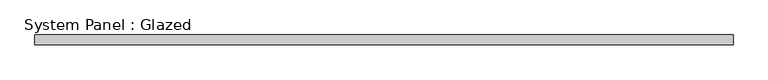
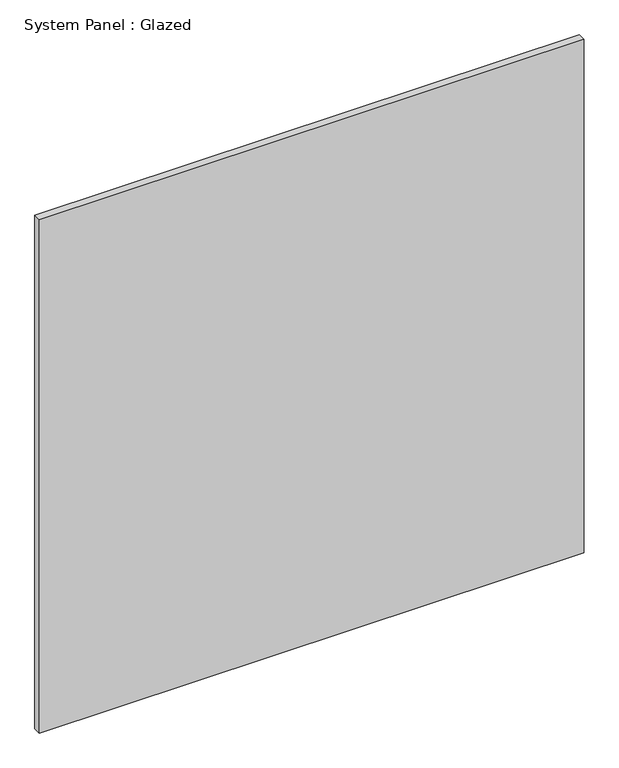
"""IFC4 building model written with IfcOpenShell, lengths in millimetres: plate geometry, System Panel : Glazed."""

from ifc_helpers import new_model, si_unit, origin, origin_with_axes, place, context, project, spatial, polyline, outline, extrude, source, transform, mapped, element, save


def system_panel_glazed_40ada530(model_context):
    return source(origin(), model_context, "Body", "SweptSolid", [
        extrude(outline(polyline([(890.0, 24.5), (-890.0, 24.5), (-890.0, 49.5), (890.0, 49.5), (890.0, 24.5)])), origin_with_axes(), (0.0, 0.0, 1.0), 1772.3836314),
    ])


if __name__ == "__main__":
    model = new_model("IFC4")
    model_context = context("Model", 3, world=origin())
    ifc_project = project(units=[si_unit("LENGTHUNIT", "METRE", prefix="MILLI")], contexts=[model_context])
    site = spatial("IfcSite", under=ifc_project)
    building = spatial("IfcBuilding", under=site)
    placement = place(None, origin())
    system_panel_glazed_shape = system_panel_glazed_40ada530(model_context)
    element("IfcPlate", 1, ObjectType="System Panel : Glazed", at=placement, inside=building, context=model_context, shape_type="MappedRepresentation", body=[
        mapped(system_panel_glazed_shape, transform((0.0, 0.0, 0.0), x_axis=(1.0, 0.0, 0.0), y_axis=(0.0, 1.0, 0.0), z_axis=(0.0, 0.0, 1.0))),
    ])
    save(model, "model.ifc")

# Revit data of these elements
# Element 1 (IfcPlate, "System Panel : Glazed")
#   Materials on its faces: "Glass"
# Materials
#   "Glass": class "Glass", colour RGB 218 227 224, transparency 0.85, Description = "Soda Lime Glass", Cost = 0
